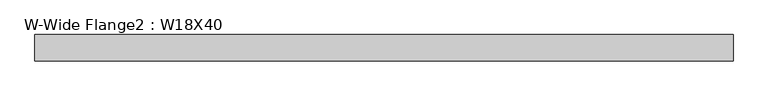
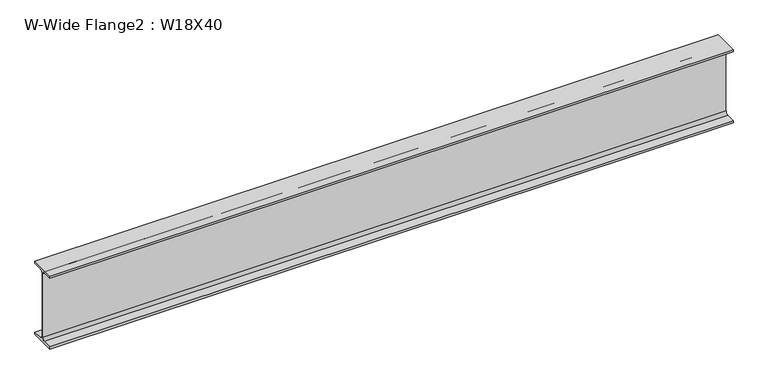
"""IFC4 building model written with IfcOpenShell, lengths in millimetres: beam geometry, W-Wide Flange2 : W18X40."""

import ifcopenshell
import ifcopenshell.guid

model = None  # the IFC model being written
_history = None  # IfcOwnerHistory: only IFC2X3 demands one
_inside = {}  # id of a spatial element -> (the spatial element, [elements in it])
_under = {}  # id of a project, library or spatial element -> (it, [spatial elements below it])
_declared = {}  # id of a project -> (the project, [libraries it declares])
_typed = {}  # id of a type object -> (the type object, [elements of that type])
_made_of = {}  # id of a material, layer set ... -> (it, [elements and type objects made of it])


def new_model(schema):
    """Start an empty IFC model of exactly this schema.

    Asked for "IFC4X3", IfcOpenShell would pick the latest addendum, in which some entities
    have other attributes; the version numbers below select the first issue.
    IFC2X3 requires an IfcOwnerHistory on every rooted entity: one is made here for all.
    """
    global model, _history
    if schema == "IFC4X3":
        model = ifcopenshell.file(schema_version=(4, 3, 0, 0))
    else:
        model = ifcopenshell.file(schema=schema)
    _inside.clear()
    _under.clear()
    _declared.clear()
    _typed.clear()
    _made_of.clear()
    _history = None
    if model.schema == "IFC2X3":
        org = make("IfcOrganization", Name="unknown")
        user = make(
            "IfcPersonAndOrganization",
            ThePerson=make("IfcPerson", FamilyName="unknown"),
            TheOrganization=org,
        )
        app = make(
            "IfcApplication",
            ApplicationDeveloper=org,
            Version="unknown",
            ApplicationFullName="unknown",
            ApplicationIdentifier="unknown",
        )
        _history = make(
            "IfcOwnerHistory",
            OwningUser=user,
            OwningApplication=app,
            ChangeAction="ADDED",
            CreationDate=0,
        )
    return model


def make(cls, **values):
    """One entity of the class cls with the attributes given. An attribute that is None is left unset."""
    return model.create_entity(
        cls, **{name: value for name, value in values.items() if value is not None}
    )


def rooted(cls, **values):
    """An entity with a GlobalId (a new one), such as an element, a storey or a relation."""
    return make(cls, GlobalId=ifcopenshell.guid.new(), OwnerHistory=_history, **values)


def si_unit(unit_type, name, prefix=None):
    """IfcSIUnit, for example si_unit("LENGTHUNIT", "METRE", prefix="MILLI")."""
    return make("IfcSIUnit", UnitType=unit_type, Prefix=prefix, Name=name)


def assignment(units):
    """IfcUnitAssignment: the units of a project."""
    return None if units is None else make("IfcUnitAssignment", Units=units)


def point(xyz):
    """IfcCartesianPoint."""
    return None if xyz is None else make("IfcCartesianPoint", Coordinates=xyz)


def direction(xyz):
    """IfcDirection."""
    return None if xyz is None else make("IfcDirection", DirectionRatios=xyz)


def frame(location, z_axis=None, x_axis=None):
    """IfcAxis2Placement3D, a coordinate frame: its origin and axes. An axis left out is left unset."""
    return make(
        "IfcAxis2Placement3D",
        Location=point(location),
        Axis=direction(z_axis),
        RefDirection=direction(x_axis),
    )


def frame_2d(location, x_axis=None):
    """IfcAxis2Placement2D, a coordinate frame in the plane: its origin and x axis."""
    return make(
        "IfcAxis2Placement2D", Location=point(location), RefDirection=direction(x_axis)
    )


def origin():
    """The frame at (0, 0, 0) with its axes left unset."""
    return frame((0.0, 0.0, 0.0))


def place(relative_to, where):
    """IfcLocalPlacement: puts the frame where relative to a parent placement (None: the world)."""
    return make(
        "IfcLocalPlacement", PlacementRelTo=relative_to, RelativePlacement=where
    )


def context(
    kind, dimensions, precision=None, world=None, true_north=None, identifier=None
):
    """IfcGeometricRepresentationContext, for example the 3D "Model" context."""
    return make(
        "IfcGeometricRepresentationContext",
        ContextIdentifier=identifier,
        ContextType=kind,
        CoordinateSpaceDimension=dimensions,
        Precision=precision,
        WorldCoordinateSystem=world,
        TrueNorth=true_north,
    )


def project(units=None, contexts=None):
    """IfcProject with its units and contexts."""
    return rooted(
        "IfcProject",
        Name="project",
        RepresentationContexts=contexts,
        UnitsInContext=assignment(units),
    )


def spatial(cls, under=None, at=None, **own):
    """A site, building, storey or space (cls), placed at a placement, below another one or the project."""
    s = rooted(cls, ObjectPlacement=at, **own)
    if under is not None:
        _under.setdefault(under.id(), (under, []))[1].append(s)
    return s


def polyline(points):
    """IfcPolyline through the points."""
    return make("IfcPolyline", Points=[point(p) for p in points])


def circle_curve(where, radius):
    """IfcCircle in the frame where."""
    return make("IfcCircle", Position=where, Radius=radius)


def trimmed(basis, trim1, trim2, sense, master):
    """IfcTrimmedCurve: the piece of a basis curve between two trims."""
    return make(
        "IfcTrimmedCurve",
        BasisCurve=basis,
        Trim1=trim1,
        Trim2=trim2,
        SenseAgreement=sense,
        MasterRepresentation=master,
    )


def segment(curve, same_sense, transition):
    """IfcCompositeCurveSegment."""
    return make(
        "IfcCompositeCurveSegment",
        Transition=transition,
        SameSense=same_sense,
        ParentCurve=curve,
    )


def composite_curve(segments, self_intersect=None):
    """IfcCompositeCurve: segments joined end to end."""
    return make("IfcCompositeCurve", Segments=segments, SelfIntersect=self_intersect)


def outline(outer, holes=None, kind="AREA"):
    """IfcArbitraryClosedProfileDef: a profile drawn as a closed curve; with holes, ...WithVoids."""
    if holes is None:
        return make("IfcArbitraryClosedProfileDef", ProfileType=kind, OuterCurve=outer)
    return make(
        "IfcArbitraryProfileDefWithVoids",
        ProfileType=kind,
        OuterCurve=outer,
        InnerCurves=holes,
    )


def extrude(swept, where, along, depth):
    """IfcExtrudedAreaSolid: the profile swept, set in the frame where, extruded along a direction by depth."""
    return make(
        "IfcExtrudedAreaSolid",
        SweptArea=swept,
        Position=where,
        ExtrudedDirection=direction(along),
        Depth=depth,
    )


def shape(context_of_items, identifier, shape_type, items):
    """IfcShapeRepresentation: the items that make up one representation, for example the "Body"."""
    return make(
        "IfcShapeRepresentation",
        ContextOfItems=context_of_items,
        RepresentationIdentifier=identifier,
        RepresentationType=shape_type,
        Items=items,
    )


def source(mapping_origin, context_of_items, identifier, shape_type, items):
    """IfcRepresentationMap: a shape defined once, which mapped items show again and again."""
    return make(
        "IfcRepresentationMap",
        MappingOrigin=mapping_origin,
        MappedRepresentation=shape(context_of_items, identifier, shape_type, items),
    )


def transform(
    local_origin,
    x_axis=None,
    y_axis=None,
    z_axis=None,
    scale=None,
    scale2=None,
    scale3=None,
    uniform=True,
):
    """IfcCartesianTransformationOperator3D, or its non-uniform kind. x_axis, y_axis, z_axis: its Axis1, 2, 3."""
    if uniform:
        return make(
            "IfcCartesianTransformationOperator3D",
            Axis1=direction(x_axis),
            Axis2=direction(y_axis),
            LocalOrigin=point(local_origin),
            Scale=scale,
            Axis3=direction(z_axis),
        )
    return make(
        "IfcCartesianTransformationOperator3DnonUniform",
        Axis1=direction(x_axis),
        Axis2=direction(y_axis),
        LocalOrigin=point(local_origin),
        Scale=scale,
        Axis3=direction(z_axis),
        Scale2=scale2,
        Scale3=scale3,
    )


def mapped(mapping_source, mapping_target):
    """IfcMappedItem: shows the shape of a source again, moved by a transform."""
    return make(
        "IfcMappedItem", MappingSource=mapping_source, MappingTarget=mapping_target
    )


def made_of(thing, what):
    """Note that an element or type object is made of a material, layer set ...; save() writes the relation."""
    if what is not None:
        _made_of.setdefault(what.id(), (what, []))[1].append(thing)
    return thing


def element(
    cls,
    number,
    at=None,
    inside=None,
    cuts=None,
    type_object=None,
    material=None,
    context=None,
    identifier="Body",
    shape_type=None,
    held_by="IfcProductDefinitionShape",
    body=None,
    shapes=None,
    **own,
):
    """One element of the class cls, such as IfcWall. Its Tag is "e" and its number.

    at: its placement. inside: the storey or other place that contains it. cuts: it is an
    opening in that element (IfcRelVoidsElement). A single representation is given by context,
    identifier, shape_type and body (its items); several are given by shapes. held_by: the class
    of the entity that holds the representations. save() writes the other relations.
    """
    e = rooted(cls, Tag="e%d" % number, ObjectPlacement=at, **own)
    if body is not None:
        shapes = [shape(context, identifier, shape_type, body)]
    if shapes is not None:
        e.Representation = make(held_by, Representations=shapes)
    if inside is not None:
        _inside.setdefault(inside.id(), (inside, []))[1].append(e)
    if cuts is not None:
        rooted(
            "IfcRelVoidsElement", RelatingBuildingElement=cuts, RelatedOpeningElement=e
        )
    if type_object is not None:
        _typed.setdefault(type_object.id(), (type_object, []))[1].append(e)
    return made_of(e, material)


def aggregate(whole, parts):
    """IfcRelAggregates: a whole, such as a stair, and the parts it consists of."""
    return rooted("IfcRelAggregates", RelatingObject=whole, RelatedObjects=parts)


def save(model, path):
    """Write the relations noted so far, then the file.

    IfcRelAggregates (storeys below a building ...), IfcRelContainedInSpatialStructure (elements
    in a storey), IfcRelDefinesByType, IfcRelAssociatesMaterial and IfcRelDeclares: one each for
    every whole, place, type object, material and project.
    """
    for whole, parts in _under.values():
        aggregate(whole, parts)
    for where, things in _inside.values():
        rooted(
            "IfcRelContainedInSpatialStructure",
            RelatedElements=things,
            RelatingStructure=where,
        )
    for kind, things in _typed.values():
        rooted("IfcRelDefinesByType", RelatedObjects=things, RelatingType=kind)
    for what, things in _made_of.values():
        rooted("IfcRelAssociatesMaterial", RelatedObjects=things, RelatingMaterial=what)
    for by, libraries in _declared.values():
        rooted("IfcRelDeclares", RelatingContext=by, RelatedDefinitions=libraries)
    model.write(path)


def w_wide_flange2_w18x40_962a7e4b(model_context):
    return source(origin(), model_context, "Body", "SweptSolid", [
        extrude(outline(composite_curve([segment(polyline([(76.454, -213.995), (76.454, -227.33), (-76.454, -227.33), (-76.454, -213.995), (-20.828, -213.995)]), True, "CONTINUOUS"), segment(trimmed(circle_curve(frame_2d((-20.828, -197.1675)), 16.8275), [point((-20.828, -213.995))], [point((-4.0005, -197.1675))], True, "CARTESIAN"), True, "CONTINUOUS"), segment(polyline([(-4.0005, -197.1675), (-4.0005, 197.1675)]), True, "CONTINUOUS"), segment(trimmed(circle_curve(frame_2d((-20.828, 197.1675)), 16.8275), [point((-4.0005, 197.1675))], [point((-20.828, 213.995))], True, "CARTESIAN"), True, "CONTINUOUS"), segment(polyline([(-20.828, 213.995), (-76.454, 213.995), (-76.454, 227.33), (76.454, 227.33), (76.454, 213.995), (20.828, 213.995)]), True, "CONTINUOUS"), segment(trimmed(circle_curve(frame_2d((20.828, 197.1675)), 16.8275), [point((20.828, 213.995))], [point((4.0005, 197.1675))], True, "CARTESIAN"), True, "CONTINUOUS"), segment(polyline([(4.0005, 197.1675), (4.0005, -197.1675)]), True, "CONTINUOUS"), segment(trimmed(circle_curve(frame_2d((20.828, -197.1675)), 16.8275), [point((4.0005, -197.1675))], [point((20.828, -213.995))], True, "CARTESIAN"), True, "CONTINUOUS"), segment(polyline([(20.828, -213.995), (76.454, -213.995)]), True, "CONTINUOUS")], self_intersect=False)), frame((-2012.553125, 0.0, 0.0), z_axis=(1.0, 0.0, 0.0), x_axis=(0.0, 1.0, 0.0)), (0.0, 0.0, 1.0), 4025.10625),
    ])


if __name__ == "__main__":
    model = new_model("IFC4")
    model_context = context("Model", 3, world=origin())
    ifc_project = project(units=[si_unit("LENGTHUNIT", "METRE", prefix="MILLI")], contexts=[model_context])
    site = spatial("IfcSite", under=ifc_project)
    building = spatial("IfcBuilding", under=site)
    placement = place(None, origin())
    w_wide_flange2_w18x40_shape = w_wide_flange2_w18x40_962a7e4b(model_context)
    element("IfcBeam", 1, ObjectType="W-Wide Flange2 : W18X40", at=placement, inside=building, context=model_context, shape_type="MappedRepresentation", body=[
        mapped(w_wide_flange2_w18x40_shape, transform((0.0, 0.0, 0.0), x_axis=(1.0, 0.0, 0.0), y_axis=(0.0, 1.0, 0.0), z_axis=(0.0, 0.0, 1.0))),
    ])
    save(model, "model.ifc")

# Revit data of these elements
# Type "W-Wide Flange2 : W18X40"
#   Assembly Code = "B10"
#   W = 40
#   Length [instance default] = 5' - 0"
#   bf = 0' - 6.02"
#   d = 1' - 5.9"
#   k = 0' - 1 3/16"
#   k2 = 0' - 0.6625"
#   tf = 0' - 0.525"
#   tw = 0' - 0.315"
#   A = 0.0819444 SF
#   Structural Material [instance default] = Steel ASTM A992
# Element 1 (IfcBeam, "W-Wide Flange2 : W18X40")
#   Materials on its faces: "Steel ASTM A992"
# Materials
#   "Steel ASTM A992": class "Metal", colour RGB 199 199 199, transparency 0, Description = "Structural steel 50ksi", Cost = 0
